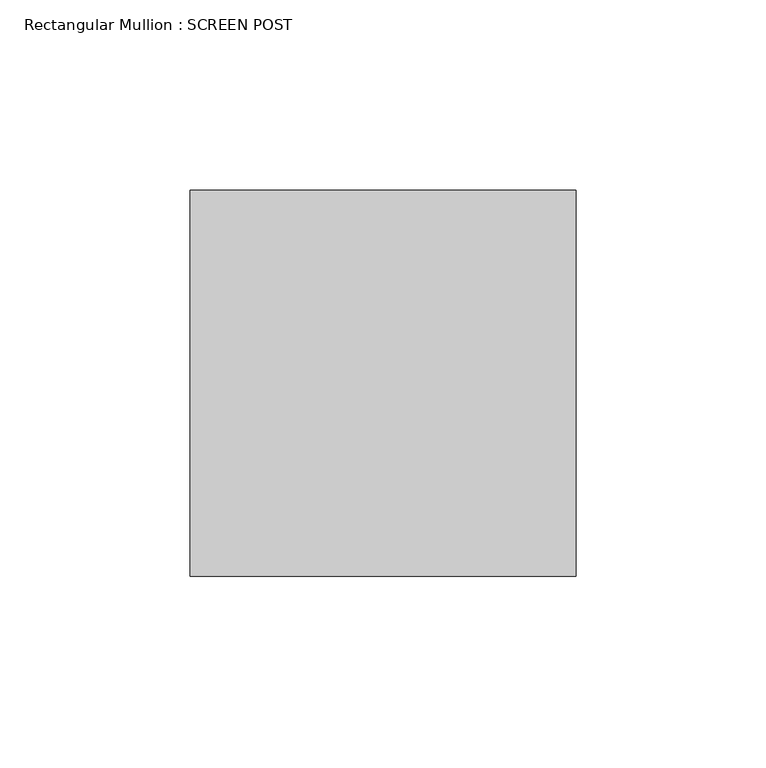
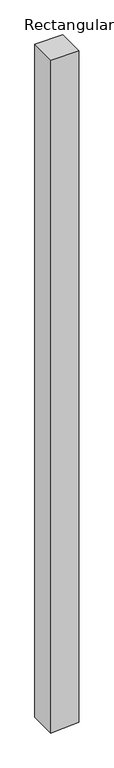
"""IFC4 building model written with IfcOpenShell, lengths in millimetres: member geometry, Rectangular Mullion : SCREEN POST."""

from ifc_helpers import new_model, si_unit, frame, origin, place, context, project, spatial, polyline, outline, extrude, source, transform, mapped, element, save


def rectangular_mullion_screen_post_282fb913(model_context):
    return source(origin(), model_context, "Body", "SweptSolid", [
        extrude(outline(polyline([(0.0, 50.8), (0.0, -50.8), (-2603.5329474, -50.8), (-2600.7497432, -6.3490391), (-2597.1714752, 50.8), (0.0, 50.8)])), frame((0.0, -50.8, 0.0), z_axis=(0.0, 1.0, 0.0), x_axis=(0.0, 0.0, 1.0)), (0.0, 0.0, 1.0), 101.6),
    ])


if __name__ == "__main__":
    model = new_model("IFC4")
    model_context = context("Model", 3, world=origin())
    ifc_project = project(units=[si_unit("LENGTHUNIT", "METRE", prefix="MILLI")], contexts=[model_context])
    site = spatial("IfcSite", under=ifc_project)
    building = spatial("IfcBuilding", under=site)
    placement = place(None, origin())
    rectangular_mullion_screen_post_shape = rectangular_mullion_screen_post_282fb913(model_context)
    element("IfcMember", 1, ObjectType="Rectangular Mullion : SCREEN POST", at=placement, inside=building, context=model_context, shape_type="MappedRepresentation", body=[
        mapped(rectangular_mullion_screen_post_shape, transform((0.0, 0.0, 0.0), x_axis=(1.0, 0.0, 0.0), y_axis=(0.0, 1.0, 0.0), z_axis=(0.0, 0.0, 1.0))),
    ])
    save(model, "model.ifc")

# Revit data of these elements
# Type "Rectangular Mullion : SCREEN POST"
#   built-in parameter 1007304 = 0.333333 (stored number, unit not read)
#   built-in parameter 1007301 = 0.166667 (stored number, unit not read)
#   built-in parameter 1007300 = 0.166667 (stored number, unit not read)
# Element 1 (IfcMember, "Rectangular Mullion : SCREEN POST")
#   Materials on its faces: "GLULAMS COLUMNS\n(PRESSURE TREATED W/ PENTA IN SOLVENT) (EXTERIOR STAIN: PENOFIN VERDE EXT. STAIN - COLOR: CEDAR)"
# Materials
#   "GLULAMS COLUMNS\n(PRESSURE TREATED W/ PENTA IN SOLVENT) (EXTERIOR STAIN: PENOFIN VERDE EXT. STAIN - COLOR: CEDAR)": class "Wood", colour RGB 164 134 123, transparency 0, Description = "Pinus Echinata", Cost = 0
